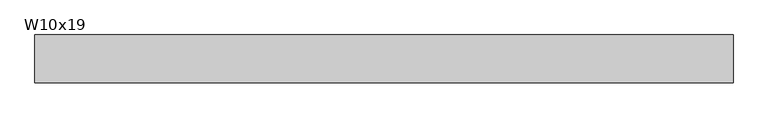
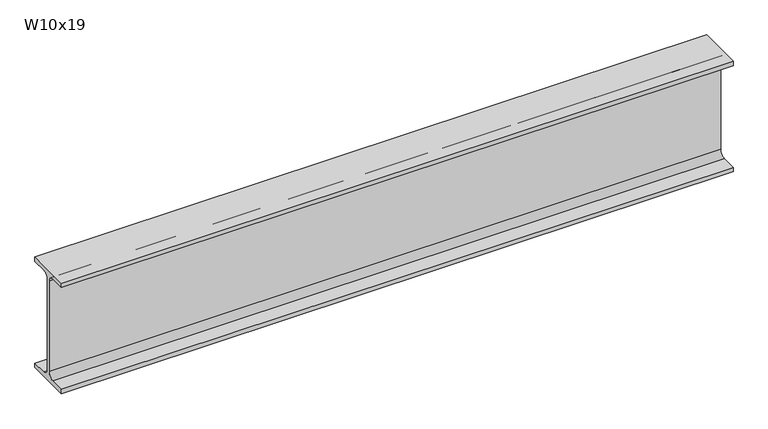
"""IFC4 building model written with IfcOpenShell, lengths in millimetres: beam geometry, RME W-Wide Flange : W10x19."""

import ifcopenshell
import ifcopenshell.guid

model = None  # the IFC model being written
_history = None  # IfcOwnerHistory: only IFC2X3 demands one
_inside = {}  # id of a spatial element -> (the spatial element, [elements in it])
_under = {}  # id of a project, library or spatial element -> (it, [spatial elements below it])
_declared = {}  # id of a project -> (the project, [libraries it declares])
_typed = {}  # id of a type object -> (the type object, [elements of that type])
_made_of = {}  # id of a material, layer set ... -> (it, [elements and type objects made of it])


def new_model(schema):
    """Start an empty IFC model of exactly this schema.

    Asked for "IFC4X3", IfcOpenShell would pick the latest addendum, in which some entities
    have other attributes; the version numbers below select the first issue.
    IFC2X3 requires an IfcOwnerHistory on every rooted entity: one is made here for all.
    """
    global model, _history
    if schema == "IFC4X3":
        model = ifcopenshell.file(schema_version=(4, 3, 0, 0))
    else:
        model = ifcopenshell.file(schema=schema)
    _inside.clear()
    _under.clear()
    _declared.clear()
    _typed.clear()
    _made_of.clear()
    _history = None
    if model.schema == "IFC2X3":
        org = make("IfcOrganization", Name="unknown")
        user = make(
            "IfcPersonAndOrganization",
            ThePerson=make("IfcPerson", FamilyName="unknown"),
            TheOrganization=org,
        )
        app = make(
            "IfcApplication",
            ApplicationDeveloper=org,
            Version="unknown",
            ApplicationFullName="unknown",
            ApplicationIdentifier="unknown",
        )
        _history = make(
            "IfcOwnerHistory",
            OwningUser=user,
            OwningApplication=app,
            ChangeAction="ADDED",
            CreationDate=0,
        )
    return model


def make(cls, **values):
    """One entity of the class cls with the attributes given. An attribute that is None is left unset."""
    return model.create_entity(
        cls, **{name: value for name, value in values.items() if value is not None}
    )


def rooted(cls, **values):
    """An entity with a GlobalId (a new one), such as an element, a storey or a relation."""
    return make(cls, GlobalId=ifcopenshell.guid.new(), OwnerHistory=_history, **values)


def si_unit(unit_type, name, prefix=None):
    """IfcSIUnit, for example si_unit("LENGTHUNIT", "METRE", prefix="MILLI")."""
    return make("IfcSIUnit", UnitType=unit_type, Prefix=prefix, Name=name)


def assignment(units):
    """IfcUnitAssignment: the units of a project."""
    return None if units is None else make("IfcUnitAssignment", Units=units)


def point(xyz):
    """IfcCartesianPoint."""
    return None if xyz is None else make("IfcCartesianPoint", Coordinates=xyz)


def direction(xyz):
    """IfcDirection."""
    return None if xyz is None else make("IfcDirection", DirectionRatios=xyz)


def frame(location, z_axis=None, x_axis=None):
    """IfcAxis2Placement3D, a coordinate frame: its origin and axes. An axis left out is left unset."""
    return make(
        "IfcAxis2Placement3D",
        Location=point(location),
        Axis=direction(z_axis),
        RefDirection=direction(x_axis),
    )


def frame_2d(location, x_axis=None):
    """IfcAxis2Placement2D, a coordinate frame in the plane: its origin and x axis."""
    return make(
        "IfcAxis2Placement2D", Location=point(location), RefDirection=direction(x_axis)
    )


def origin():
    """The frame at (0, 0, 0) with its axes left unset."""
    return frame((0.0, 0.0, 0.0))


def place(relative_to, where):
    """IfcLocalPlacement: puts the frame where relative to a parent placement (None: the world)."""
    return make(
        "IfcLocalPlacement", PlacementRelTo=relative_to, RelativePlacement=where
    )


def context(
    kind, dimensions, precision=None, world=None, true_north=None, identifier=None
):
    """IfcGeometricRepresentationContext, for example the 3D "Model" context."""
    return make(
        "IfcGeometricRepresentationContext",
        ContextIdentifier=identifier,
        ContextType=kind,
        CoordinateSpaceDimension=dimensions,
        Precision=precision,
        WorldCoordinateSystem=world,
        TrueNorth=true_north,
    )


def project(units=None, contexts=None):
    """IfcProject with its units and contexts."""
    return rooted(
        "IfcProject",
        Name="project",
        RepresentationContexts=contexts,
        UnitsInContext=assignment(units),
    )


def spatial(cls, under=None, at=None, **own):
    """A site, building, storey or space (cls), placed at a placement, below another one or the project."""
    s = rooted(cls, ObjectPlacement=at, **own)
    if under is not None:
        _under.setdefault(under.id(), (under, []))[1].append(s)
    return s


def polyline(points):
    """IfcPolyline through the points."""
    return make("IfcPolyline", Points=[point(p) for p in points])


def circle_curve(where, radius):
    """IfcCircle in the frame where."""
    return make("IfcCircle", Position=where, Radius=radius)


def trimmed(basis, trim1, trim2, sense, master):
    """IfcTrimmedCurve: the piece of a basis curve between two trims."""
    return make(
        "IfcTrimmedCurve",
        BasisCurve=basis,
        Trim1=trim1,
        Trim2=trim2,
        SenseAgreement=sense,
        MasterRepresentation=master,
    )


def segment(curve, same_sense, transition):
    """IfcCompositeCurveSegment."""
    return make(
        "IfcCompositeCurveSegment",
        Transition=transition,
        SameSense=same_sense,
        ParentCurve=curve,
    )


def composite_curve(segments, self_intersect=None):
    """IfcCompositeCurve: segments joined end to end."""
    return make("IfcCompositeCurve", Segments=segments, SelfIntersect=self_intersect)


def outline(outer, holes=None, kind="AREA"):
    """IfcArbitraryClosedProfileDef: a profile drawn as a closed curve; with holes, ...WithVoids."""
    if holes is None:
        return make("IfcArbitraryClosedProfileDef", ProfileType=kind, OuterCurve=outer)
    return make(
        "IfcArbitraryProfileDefWithVoids",
        ProfileType=kind,
        OuterCurve=outer,
        InnerCurves=holes,
    )


def extrude(swept, where, along, depth):
    """IfcExtrudedAreaSolid: the profile swept, set in the frame where, extruded along a direction by depth."""
    return make(
        "IfcExtrudedAreaSolid",
        SweptArea=swept,
        Position=where,
        ExtrudedDirection=direction(along),
        Depth=depth,
    )


def shape(context_of_items, identifier, shape_type, items):
    """IfcShapeRepresentation: the items that make up one representation, for example the "Body"."""
    return make(
        "IfcShapeRepresentation",
        ContextOfItems=context_of_items,
        RepresentationIdentifier=identifier,
        RepresentationType=shape_type,
        Items=items,
    )


def source(mapping_origin, context_of_items, identifier, shape_type, items):
    """IfcRepresentationMap: a shape defined once, which mapped items show again and again."""
    return make(
        "IfcRepresentationMap",
        MappingOrigin=mapping_origin,
        MappedRepresentation=shape(context_of_items, identifier, shape_type, items),
    )


def transform(
    local_origin,
    x_axis=None,
    y_axis=None,
    z_axis=None,
    scale=None,
    scale2=None,
    scale3=None,
    uniform=True,
):
    """IfcCartesianTransformationOperator3D, or its non-uniform kind. x_axis, y_axis, z_axis: its Axis1, 2, 3."""
    if uniform:
        return make(
            "IfcCartesianTransformationOperator3D",
            Axis1=direction(x_axis),
            Axis2=direction(y_axis),
            LocalOrigin=point(local_origin),
            Scale=scale,
            Axis3=direction(z_axis),
        )
    return make(
        "IfcCartesianTransformationOperator3DnonUniform",
        Axis1=direction(x_axis),
        Axis2=direction(y_axis),
        LocalOrigin=point(local_origin),
        Scale=scale,
        Axis3=direction(z_axis),
        Scale2=scale2,
        Scale3=scale3,
    )


def mapped(mapping_source, mapping_target):
    """IfcMappedItem: shows the shape of a source again, moved by a transform."""
    return make(
        "IfcMappedItem", MappingSource=mapping_source, MappingTarget=mapping_target
    )


def made_of(thing, what):
    """Note that an element or type object is made of a material, layer set ...; save() writes the relation."""
    if what is not None:
        _made_of.setdefault(what.id(), (what, []))[1].append(thing)
    return thing


def element(
    cls,
    number,
    at=None,
    inside=None,
    cuts=None,
    type_object=None,
    material=None,
    context=None,
    identifier="Body",
    shape_type=None,
    held_by="IfcProductDefinitionShape",
    body=None,
    shapes=None,
    **own,
):
    """One element of the class cls, such as IfcWall. Its Tag is "e" and its number.

    at: its placement. inside: the storey or other place that contains it. cuts: it is an
    opening in that element (IfcRelVoidsElement). A single representation is given by context,
    identifier, shape_type and body (its items); several are given by shapes. held_by: the class
    of the entity that holds the representations. save() writes the other relations.
    """
    e = rooted(cls, Tag="e%d" % number, ObjectPlacement=at, **own)
    if body is not None:
        shapes = [shape(context, identifier, shape_type, body)]
    if shapes is not None:
        e.Representation = make(held_by, Representations=shapes)
    if inside is not None:
        _inside.setdefault(inside.id(), (inside, []))[1].append(e)
    if cuts is not None:
        rooted(
            "IfcRelVoidsElement", RelatingBuildingElement=cuts, RelatedOpeningElement=e
        )
    if type_object is not None:
        _typed.setdefault(type_object.id(), (type_object, []))[1].append(e)
    return made_of(e, material)


def aggregate(whole, parts):
    """IfcRelAggregates: a whole, such as a stair, and the parts it consists of."""
    return rooted("IfcRelAggregates", RelatingObject=whole, RelatedObjects=parts)


def save(model, path):
    """Write the relations noted so far, then the file.

    IfcRelAggregates (storeys below a building ...), IfcRelContainedInSpatialStructure (elements
    in a storey), IfcRelDefinesByType, IfcRelAssociatesMaterial and IfcRelDeclares: one each for
    every whole, place, type object, material and project.
    """
    for whole, parts in _under.values():
        aggregate(whole, parts)
    for where, things in _inside.values():
        rooted(
            "IfcRelContainedInSpatialStructure",
            RelatedElements=things,
            RelatingStructure=where,
        )
    for kind, things in _typed.values():
        rooted("IfcRelDefinesByType", RelatedObjects=things, RelatingType=kind)
    for what, things in _made_of.values():
        rooted("IfcRelAssociatesMaterial", RelatedObjects=things, RelatingMaterial=what)
    for by, libraries in _declared.values():
        rooted("IfcRelDeclares", RelatingContext=by, RelatedDefinitions=libraries)
    model.write(path)


def w10x19_6627e6d8(model_context):
    return source(origin(), model_context, "Body", "SweptSolid", [
        extrude(outline(composite_curve([segment(polyline([(51.054, -119.507), (51.054, -129.54), (-51.054, -129.54), (-51.054, -119.507), (-16.9545, -119.507)]), True, "CONTINUOUS"), segment(trimmed(circle_curve(frame_2d((-16.9545, -105.7275)), 13.7795), [point((-16.9545, -119.507))], [point((-3.175, -105.7275))], True, "CARTESIAN"), True, "CONTINUOUS"), segment(polyline([(-3.175, -105.7275), (-3.175, 105.7275)]), True, "CONTINUOUS"), segment(trimmed(circle_curve(frame_2d((-16.9545, 105.7275)), 13.7795), [point((-3.175, 105.7275))], [point((-16.9545, 119.507))], True, "CARTESIAN"), True, "CONTINUOUS"), segment(polyline([(-16.9545, 119.507), (-51.054, 119.507), (-51.054, 129.54), (51.054, 129.54), (51.054, 119.507), (16.9545, 119.507)]), True, "CONTINUOUS"), segment(trimmed(circle_curve(frame_2d((16.9545, 105.7275)), 13.7795), [point((16.9545, 119.507))], [point((3.175, 105.7275))], True, "CARTESIAN"), True, "CONTINUOUS"), segment(polyline([(3.175, 105.7275), (3.175, -105.7275)]), True, "CONTINUOUS"), segment(trimmed(circle_curve(frame_2d((16.9545, -105.7275)), 13.7795), [point((3.175, -105.7275))], [point((16.9545, -119.507))], True, "CARTESIAN"), True, "CONTINUOUS"), segment(polyline([(16.9545, -119.507), (51.054, -119.507)]), True, "CONTINUOUS")], self_intersect=False)), frame((-713.1019715, 0.0, 0.0), z_axis=(1.0, 0.0, 0.0), x_axis=(0.0, 1.0, 0.0)), (0.0, 0.0, 1.0), 1489.703943),
    ])


if __name__ == "__main__":
    model = new_model("IFC4")
    model_context = context("Model", 3, world=origin())
    ifc_project = project(units=[si_unit("LENGTHUNIT", "METRE", prefix="MILLI")], contexts=[model_context])
    site = spatial("IfcSite", under=ifc_project)
    building = spatial("IfcBuilding", under=site)
    placement = place(None, origin())
    w10x19_shape = w10x19_6627e6d8(model_context)
    element("IfcBeam", 1, ObjectType="RME W-Wide Flange : W10x19", at=placement, inside=building, context=model_context, shape_type="MappedRepresentation", body=[
        mapped(w10x19_shape, transform((0.0, 0.0, 0.0), x_axis=(1.0, 0.0, 0.0), y_axis=(0.0, 1.0, 0.0), z_axis=(0.0, 0.0, 1.0))),
    ])
    save(model, "model.ifc")

# Revit data of these elements
# Type "RME W-Wide Flange : W10x19"
#   WELD P [instance default] = ""
#   WELD LE [instance default] = ""
#   WELD D [instance default] = ""
#   TOP SECTION SIZE [instance default] = ""
#   TOP SECTION LENGTH [instance default] = ""
#   REMARKS [instance default] = ""
#   REINF TYPE [instance default] = ""
#   Nominal Size = "W24"
#   End Bearing Capacity [instance default] = ""
#   BOT SECTION SIZE [instance default] = ""
#   BOT SECTION LENGTH [instance default] = ""
#   Assembly Code = "B10"
#   W = 19
#   Start Extension Calculation [instance default] = 10' - 0"
#   Start Extension [instance default] = -0' - 0 1/2"
#   End Extension Calculation [instance default] = 10' - 0"
#   End Extension [instance default] = -0' - 0 1/2"
#   Length [instance default] = 5' - 0"
#   bf = 0' - 4.02"
#   d = 0' - 10.2"
#   k = 0' - 0 15/16"
#   k2 = 0' - 0.5425"
#   tf = 0' - 0.395"
#   tw = 0' - 0 1/4"
#   A = 0.0390278 SF
#   Structural Material [instance default] = Metal - Steel - ASTM A992
# Element 1 (IfcBeam, "RME W-Wide Flange : W10x19")
#   Length = 5' - 1.14976"
#   Materials on its faces: "Metal - Steel - ASTM A992"
# Materials
#   "Metal - Steel - ASTM A992": class "Metal", colour RGB 255 128 0, transparency 0
